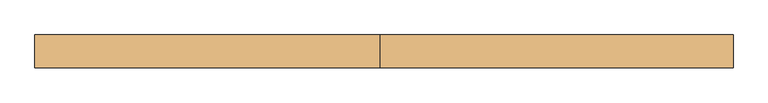
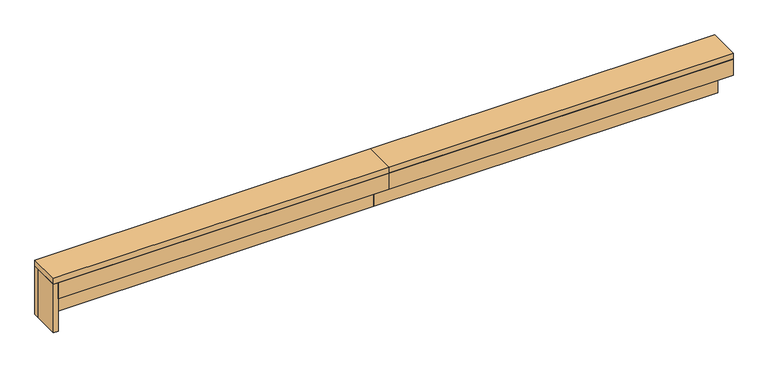
"""IFC4 building model written with IfcOpenShell, lengths in millimetres: door geometry, Schiebetür."""

import ifcopenshell
import ifcopenshell.guid

model = None  # the IFC model being written
_history = None  # IfcOwnerHistory: only IFC2X3 demands one
_inside = {}  # id of a spatial element -> (the spatial element, [elements in it])
_under = {}  # id of a project, library or spatial element -> (it, [spatial elements below it])
_declared = {}  # id of a project -> (the project, [libraries it declares])
_typed = {}  # id of a type object -> (the type object, [elements of that type])
_made_of = {}  # id of a material, layer set ... -> (it, [elements and type objects made of it])


def new_model(schema):
    """Start an empty IFC model of exactly this schema.

    Asked for "IFC4X3", IfcOpenShell would pick the latest addendum, in which some entities
    have other attributes; the version numbers below select the first issue.
    IFC2X3 requires an IfcOwnerHistory on every rooted entity: one is made here for all.
    """
    global model, _history
    if schema == "IFC4X3":
        model = ifcopenshell.file(schema_version=(4, 3, 0, 0))
    else:
        model = ifcopenshell.file(schema=schema)
    _inside.clear()
    _under.clear()
    _declared.clear()
    _typed.clear()
    _made_of.clear()
    _history = None
    if model.schema == "IFC2X3":
        org = make("IfcOrganization", Name="unknown")
        user = make(
            "IfcPersonAndOrganization",
            ThePerson=make("IfcPerson", FamilyName="unknown"),
            TheOrganization=org,
        )
        app = make(
            "IfcApplication",
            ApplicationDeveloper=org,
            Version="unknown",
            ApplicationFullName="unknown",
            ApplicationIdentifier="unknown",
        )
        _history = make(
            "IfcOwnerHistory",
            OwningUser=user,
            OwningApplication=app,
            ChangeAction="ADDED",
            CreationDate=0,
        )
    return model


def make(cls, **values):
    """One entity of the class cls with the attributes given. An attribute that is None is left unset."""
    return model.create_entity(
        cls, **{name: value for name, value in values.items() if value is not None}
    )


def rooted(cls, **values):
    """An entity with a GlobalId (a new one), such as an element, a storey or a relation."""
    return make(cls, GlobalId=ifcopenshell.guid.new(), OwnerHistory=_history, **values)


def si_unit(unit_type, name, prefix=None):
    """IfcSIUnit, for example si_unit("LENGTHUNIT", "METRE", prefix="MILLI")."""
    return make("IfcSIUnit", UnitType=unit_type, Prefix=prefix, Name=name)


def assignment(units):
    """IfcUnitAssignment: the units of a project."""
    return None if units is None else make("IfcUnitAssignment", Units=units)


def point(xyz):
    """IfcCartesianPoint."""
    return None if xyz is None else make("IfcCartesianPoint", Coordinates=xyz)


def direction(xyz):
    """IfcDirection."""
    return None if xyz is None else make("IfcDirection", DirectionRatios=xyz)


def frame(location, z_axis=None, x_axis=None):
    """IfcAxis2Placement3D, a coordinate frame: its origin and axes. An axis left out is left unset."""
    return make(
        "IfcAxis2Placement3D",
        Location=point(location),
        Axis=direction(z_axis),
        RefDirection=direction(x_axis),
    )


def origin():
    """The frame at (0, 0, 0) with its axes left unset."""
    return frame((0.0, 0.0, 0.0))


def origin_with_axes():
    """The frame at (0, 0, 0) with the z axis (0, 0, 1) and the x axis (1, 0, 0) written out."""
    return frame((0.0, 0.0, 0.0), z_axis=(0.0, 0.0, 1.0), x_axis=(1.0, 0.0, 0.0))


def place(relative_to, where):
    """IfcLocalPlacement: puts the frame where relative to a parent placement (None: the world)."""
    return make(
        "IfcLocalPlacement", PlacementRelTo=relative_to, RelativePlacement=where
    )


def context(
    kind, dimensions, precision=None, world=None, true_north=None, identifier=None
):
    """IfcGeometricRepresentationContext, for example the 3D "Model" context."""
    return make(
        "IfcGeometricRepresentationContext",
        ContextIdentifier=identifier,
        ContextType=kind,
        CoordinateSpaceDimension=dimensions,
        Precision=precision,
        WorldCoordinateSystem=world,
        TrueNorth=true_north,
    )


def project(units=None, contexts=None):
    """IfcProject with its units and contexts."""
    return rooted(
        "IfcProject",
        Name="project",
        RepresentationContexts=contexts,
        UnitsInContext=assignment(units),
    )


def spatial(cls, under=None, at=None, **own):
    """A site, building, storey or space (cls), placed at a placement, below another one or the project."""
    s = rooted(cls, ObjectPlacement=at, **own)
    if under is not None:
        _under.setdefault(under.id(), (under, []))[1].append(s)
    return s


def polyline(points):
    """IfcPolyline through the points."""
    return make("IfcPolyline", Points=[point(p) for p in points])


def outline(outer, holes=None, kind="AREA"):
    """IfcArbitraryClosedProfileDef: a profile drawn as a closed curve; with holes, ...WithVoids."""
    if holes is None:
        return make("IfcArbitraryClosedProfileDef", ProfileType=kind, OuterCurve=outer)
    return make(
        "IfcArbitraryProfileDefWithVoids",
        ProfileType=kind,
        OuterCurve=outer,
        InnerCurves=holes,
    )


def extrude(swept, where, along, depth):
    """IfcExtrudedAreaSolid: the profile swept, set in the frame where, extruded along a direction by depth."""
    return make(
        "IfcExtrudedAreaSolid",
        SweptArea=swept,
        Position=where,
        ExtrudedDirection=direction(along),
        Depth=depth,
    )


def shape(context_of_items, identifier, shape_type, items):
    """IfcShapeRepresentation: the items that make up one representation, for example the "Body"."""
    return make(
        "IfcShapeRepresentation",
        ContextOfItems=context_of_items,
        RepresentationIdentifier=identifier,
        RepresentationType=shape_type,
        Items=items,
    )


def source(mapping_origin, context_of_items, identifier, shape_type, items):
    """IfcRepresentationMap: a shape defined once, which mapped items show again and again."""
    return make(
        "IfcRepresentationMap",
        MappingOrigin=mapping_origin,
        MappedRepresentation=shape(context_of_items, identifier, shape_type, items),
    )


def transform(
    local_origin,
    x_axis=None,
    y_axis=None,
    z_axis=None,
    scale=None,
    scale2=None,
    scale3=None,
    uniform=True,
):
    """IfcCartesianTransformationOperator3D, or its non-uniform kind. x_axis, y_axis, z_axis: its Axis1, 2, 3."""
    if uniform:
        return make(
            "IfcCartesianTransformationOperator3D",
            Axis1=direction(x_axis),
            Axis2=direction(y_axis),
            LocalOrigin=point(local_origin),
            Scale=scale,
            Axis3=direction(z_axis),
        )
    return make(
        "IfcCartesianTransformationOperator3DnonUniform",
        Axis1=direction(x_axis),
        Axis2=direction(y_axis),
        LocalOrigin=point(local_origin),
        Scale=scale,
        Axis3=direction(z_axis),
        Scale2=scale2,
        Scale3=scale3,
    )


def mapped(mapping_source, mapping_target):
    """IfcMappedItem: shows the shape of a source again, moved by a transform."""
    return make(
        "IfcMappedItem", MappingSource=mapping_source, MappingTarget=mapping_target
    )


def made_of(thing, what):
    """Note that an element or type object is made of a material, layer set ...; save() writes the relation."""
    if what is not None:
        _made_of.setdefault(what.id(), (what, []))[1].append(thing)
    return thing


def element(
    cls,
    number,
    at=None,
    inside=None,
    cuts=None,
    type_object=None,
    material=None,
    context=None,
    identifier="Body",
    shape_type=None,
    held_by="IfcProductDefinitionShape",
    body=None,
    shapes=None,
    **own,
):
    """One element of the class cls, such as IfcWall. Its Tag is "e" and its number.

    at: its placement. inside: the storey or other place that contains it. cuts: it is an
    opening in that element (IfcRelVoidsElement). A single representation is given by context,
    identifier, shape_type and body (its items); several are given by shapes. held_by: the class
    of the entity that holds the representations. save() writes the other relations.
    """
    e = rooted(cls, Tag="e%d" % number, ObjectPlacement=at, **own)
    if body is not None:
        shapes = [shape(context, identifier, shape_type, body)]
    if shapes is not None:
        e.Representation = make(held_by, Representations=shapes)
    if inside is not None:
        _inside.setdefault(inside.id(), (inside, []))[1].append(e)
    if cuts is not None:
        rooted(
            "IfcRelVoidsElement", RelatingBuildingElement=cuts, RelatedOpeningElement=e
        )
    if type_object is not None:
        _typed.setdefault(type_object.id(), (type_object, []))[1].append(e)
    return made_of(e, material)


def aggregate(whole, parts):
    """IfcRelAggregates: a whole, such as a stair, and the parts it consists of."""
    return rooted("IfcRelAggregates", RelatingObject=whole, RelatedObjects=parts)


def save(model, path):
    """Write the relations noted so far, then the file.

    IfcRelAggregates (storeys below a building ...), IfcRelContainedInSpatialStructure (elements
    in a storey), IfcRelDefinesByType, IfcRelAssociatesMaterial and IfcRelDeclares: one each for
    every whole, place, type object, material and project.
    """
    for whole, parts in _under.values():
        aggregate(whole, parts)
    for where, things in _inside.values():
        rooted(
            "IfcRelContainedInSpatialStructure",
            RelatedElements=things,
            RelatingStructure=where,
        )
    for kind, things in _typed.values():
        rooted("IfcRelDefinesByType", RelatedObjects=things, RelatingType=kind)
    for what, things in _made_of.values():
        rooted("IfcRelAssociatesMaterial", RelatedObjects=things, RelatingMaterial=what)
    for by, libraries in _declared.values():
        rooted("IfcRelDeclares", RelatingContext=by, RelatedDefinitions=libraries)
    model.write(path)


def door_0f05f645(model_context):
    return source(origin(), model_context, "Body", "SweptSolid", [
        extrude(outline(polyline([(1704.4507425, 0.0), (1704.4507425, -13.7142857), (841.4507425, -13.7142857), (841.4507425, 0.0), (1704.4507425, 0.0)])), origin_with_axes(), (0.0, 0.0, 1.0), 128.9099526),
        extrude(outline(polyline([(0.0, -80.0), (0.0, 0.0), (841.4507425, 0.0), (841.4507425, -80.0), (0.0, -80.0)])), frame((0.0, 0.0, 128.9099526), z_axis=(0.0, 0.0, 1.0), x_axis=(1.0, 0.0, 0.0)), (0.0, 0.0, 1.0), 15.4691943),
        extrude(outline(polyline([(12.0, -80.0), (12.0, -61.7142857), (841.4507425, -61.7142857), (841.4507425, -80.0), (12.0, -80.0)])), frame((0.0, 0.0, 86.3696682), z_axis=(0.0, 0.0, 1.0), x_axis=(1.0, 0.0, 0.0)), (0.0, 0.0, 1.0), 42.5402844),
        extrude(outline(polyline([(1704.4507425, -61.7142857), (1704.4507425, -80.0), (841.4507425, -80.0), (841.4507425, -61.7142857), (1704.4507425, -61.7142857)])), frame((0.0, 0.0, 86.3696682), z_axis=(0.0, 0.0, 1.0), x_axis=(1.0, 0.0, 0.0)), (0.0, 0.0, 1.0), 42.5402844),
        extrude(outline(polyline([(1704.4507425, 0.0), (1704.4507425, -80.0), (841.4507425, -80.0), (841.4507425, 0.0), (1704.4507425, 0.0)])), frame((0.0, 0.0, 128.9099526), z_axis=(0.0, 0.0, 1.0), x_axis=(1.0, 0.0, 0.0)), (0.0, 0.0, 1.0), 15.4691943),
        extrude(outline(polyline([(0.0, -13.7142857), (12.0, -13.7142857), (12.0, -80.0), (0.0, -80.0), (0.0, -13.7142857)])), origin_with_axes(), (0.0, 0.0, 1.0), 128.9099526),
        extrude(outline(polyline([(0.0, -13.7142857), (0.0, 0.0), (841.4507425, 0.0), (841.4507425, -13.7142857), (0.0, -13.7142857)])), origin_with_axes(), (0.0, 0.0, 1.0), 128.9099526),
    ])


if __name__ == "__main__":
    model = new_model("IFC4")
    model_context = context("Model", 3, world=origin())
    ifc_project = project(units=[si_unit("LENGTHUNIT", "METRE", prefix="MILLI")], contexts=[model_context])
    site = spatial("IfcSite", under=ifc_project)
    building = spatial("IfcBuilding", under=site)
    placement = place(None, origin())
    door_shape = door_0f05f645(model_context)
    element("IfcDoor", 1, ObjectType="Schiebetür", at=placement, inside=building, context=model_context, shape_type="MappedRepresentation", body=[
        mapped(door_shape, transform((0.0, 0.0, 0.0), x_axis=(1.0, 0.0, 0.0), y_axis=(0.0, 1.0, 0.0), z_axis=(0.0, 0.0, 1.0))),
    ])
    save(model, "model.ifc")

# Revit data of these elements
# Type "Schiebetür"
#   Type Mark = "50"
# Element 1 (IfcDoor, "Schiebetür")
#   Materials on its faces: "tuer_holzzarge"
# Materials
#   "tuer_holzzarge": class "Unassigned", colour RGB 255 255 255, transparency 0
